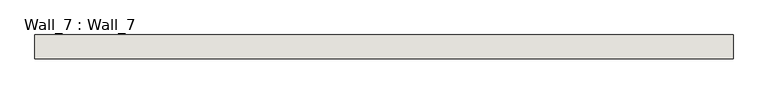
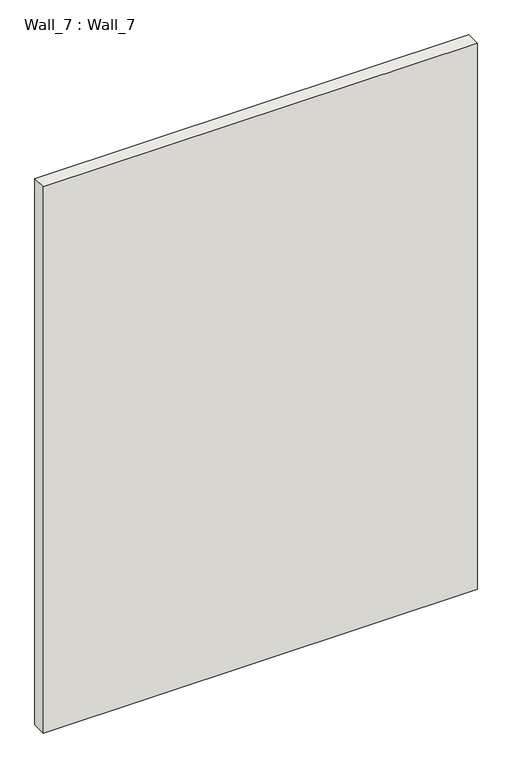
"""IFC4 building model written with IfcOpenShell, lengths in millimetres: wall geometry, Wall_7 : Wall_7."""

from ifc_helpers import new_model, si_unit, origin, origin_with_axes, place, context, project, spatial, polyline, outline, extrude, source, transform, mapped, element, save


def wall_7_wall_7_843a4671(model_context):
    return source(origin(), model_context, "Body", "SweptSolid", [
        extrude(outline(polyline([(6190.0, 16870.0), (2660.0, 16870.0), (2660.0, 16990.0), (6190.0, 16990.0), (6190.0, 16870.0)])), origin_with_axes(), (0.0, 0.0, 1.0), 4700.0),
    ])


if __name__ == "__main__":
    model = new_model("IFC4")
    model_context = context("Model", 3, world=origin())
    ifc_project = project(units=[si_unit("LENGTHUNIT", "METRE", prefix="MILLI")], contexts=[model_context])
    site = spatial("IfcSite", under=ifc_project)
    building = spatial("IfcBuilding", under=site)
    placement = place(None, origin())
    wall_7_wall_7_shape = wall_7_wall_7_843a4671(model_context)
    element("IfcWall", 1, ObjectType="Wall_7 : Wall_7", at=placement, inside=building, context=model_context, shape_type="MappedRepresentation", body=[
        mapped(wall_7_wall_7_shape, transform((0.0, 0.0, 0.0), x_axis=(1.0, 0.0, 0.0), y_axis=(0.0, 1.0, 0.0), z_axis=(0.0, 0.0, 1.0))),
    ])
    save(model, "model.ifc")

# Revit data of these elements
# Type "Wall_7 : Wall_7"
#   NameOverride = "Wall_7"
# Element 1 (IfcWall, "Wall_7 : Wall_7")
#   Materials on its faces: "IfcSurfaceStyle #33"
# Materials
#   "IfcSurfaceStyle #33": class "Unassigned", colour RGB 214 214 214, transparency 0
